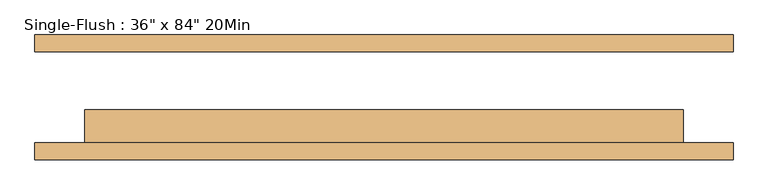
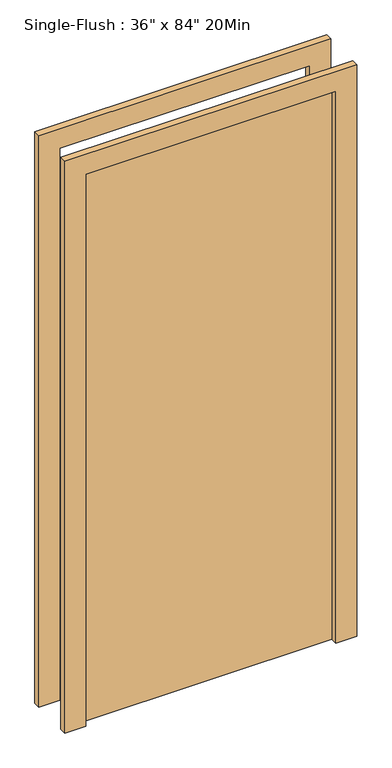
"""IFC4 building model written with IfcOpenShell, lengths in millimetres: door geometry."""

from ifc_helpers import new_model, si_unit, frame, origin, origin_with_axes, place, context, project, spatial, polyline, outline, extrude, source, transform, mapped, element, save


def door_9814c99b(model_context):
    return source(origin(), model_context, "Body", "SweptSolid", [
        extrude(outline(polyline([(2209.8, -533.4), (0.0, -533.4), (0.0, -457.2), (2133.6, -457.2), (2133.6, 457.2), (0.0, 457.2), (0.0, 533.4), (2209.8, 533.4), (2209.8, -533.4)])), frame((0.0, -95.25, 0.0), z_axis=(0.0, 1.0, 0.0), x_axis=(0.0, 0.0, 1.0)), (0.0, 0.0, 1.0), 25.4),
        extrude(outline(polyline([(2209.8, 533.4), (2209.8, -533.4), (0.0, -533.4), (0.0, -457.2), (2133.6, -457.2), (2133.6, 457.2), (0.0, 457.2), (0.0, 533.4), (2209.8, 533.4)])), frame((0.0, 69.85, 0.0), z_axis=(0.0, 1.0, 0.0), x_axis=(0.0, 0.0, 1.0)), (0.0, 0.0, 1.0), 25.4),
        extrude(outline(polyline([(457.2, -19.05), (457.2, -69.85), (-457.2, -69.85), (-457.2, -19.05), (457.2, -19.05)])), origin_with_axes(), (0.0, 0.0, 1.0), 2133.6),
    ])


if __name__ == "__main__":
    model = new_model("IFC4")
    model_context = context("Model", 3, world=origin())
    ifc_project = project(units=[si_unit("LENGTHUNIT", "METRE", prefix="MILLI")], contexts=[model_context])
    site = spatial("IfcSite", under=ifc_project)
    building = spatial("IfcBuilding", under=site)
    placement = place(None, origin())
    door_shape = door_9814c99b(model_context)
    element("IfcDoor", 1, ObjectType="Single-Flush : 36\" x 84\" 20Min", at=placement, inside=building, context=model_context, shape_type="MappedRepresentation", body=[
        mapped(door_shape, transform((0.0, 0.0, 0.0), x_axis=(1.0, 0.0, 0.0), y_axis=(0.0, 1.0, 0.0), z_axis=(0.0, 0.0, 1.0))),
    ])
    save(model, "model.ifc")

# Revit data of these elements
# Type "Single-Flush : 36\" x 84\" 20Min"
#   Type Mark = "23"
#   Fire Rating = "20 Min."
#   Assembly Code = "C1020"
#   Thickness = 50.8 mm
#   Height = 2133.6 mm
#   Trim Projection Ext = 25.4 mm
#   Trim Projection Int = 25.4 mm
#   Trim Width = 76.2 mm
#   Width = 914.4 mm
#   Define Thermal Properties by = 0
#   Door Material = Door - Panel
#   Frame Material = Door - Frame
#   Function = (empty or 0)
#   Wall Closure = (empty or 0)
# Element 1 (IfcDoor, "Single-Flush : 36\" x 84\" 20Min")
#   Materials on its faces: "Door - Frame", "Door - Panel"
# Materials
#   "Door - Panel": class "Wood", colour RGB 210 159 95, transparency 0, Cost = 0
#   "Door - Frame": class "Miscellaneous", colour RGB 118 70 51, transparency 0, Cost = 0
